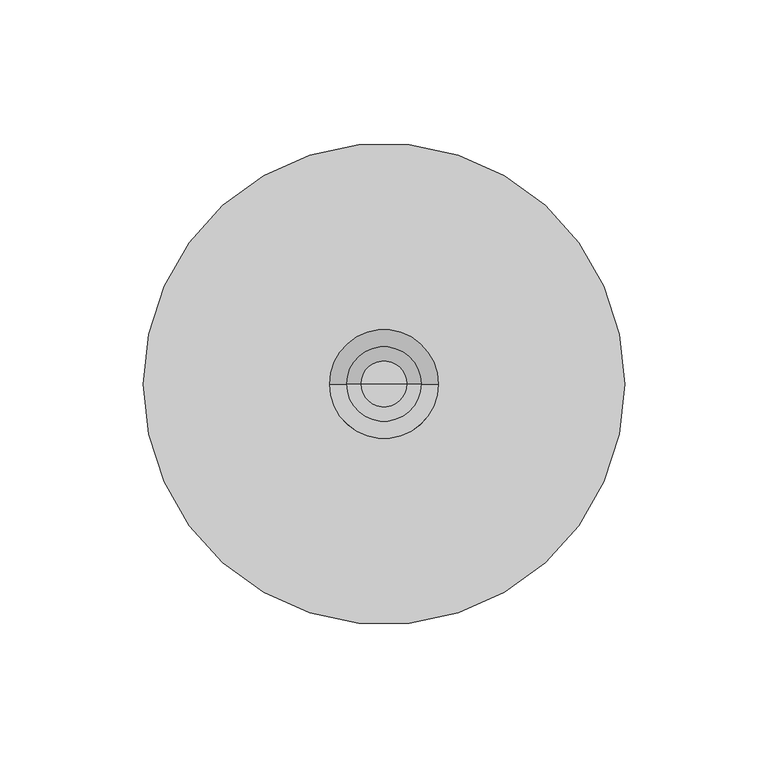
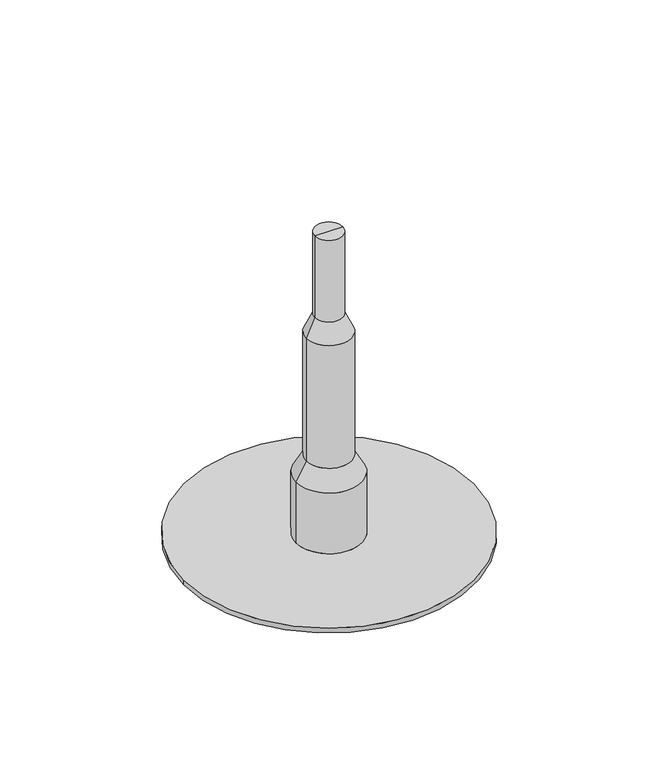
"""IFC4 building model written with IfcOpenShell, lengths in millimetres: proxy geometry, TN_Штуцер инъекционный_Прямой : ПВХ Штуцер инъекционный прямой."""

from ifc_helpers import new_model, si_unit, frame, origin, origin_with_axes, place, context, project, spatial, polyline, circle_curve, source, transform, mapped, element, save
from ifc_brep_helpers import plane_surface, cylinder_surface, revolved_surface, advanced_brep


def specialty_equipment_220ff5bd(model_context):
    return source(origin(), model_context, "Body", "AdvancedBrep", [
        advanced_brep(
        [(-19.0, 0.0, 3.0), (-19.0, 0.0, 40.0), (19.0, 0.0, 40.0), (19.0, 0.0, 3.0), (8.0, 0.0, 187.0), (-8.0, 0.0, 187.0), (0.0, 0.0, 187.0), (8.0, 0.0, 137.0), (-8.0, 0.0, 137.0), (13.0, 0.0, 126.0), (-13.0, 0.0, 126.0), (13.0, 0.0, 51.0), (-13.0, 0.0, 51.0), (-84.0, 0.0, 3.0), (84.0, 0.0, 3.0), (-84.0, 0.0, 0.0), (84.0, 0.0, 0.0)],
        [
            (0, 1),
            (1, 2, circle_curve(frame((0.0, 0.0, 40.0), z_axis=(0.0, 0.0, -1.0), x_axis=(-1.0, 0.0, 0.0)), 19.0)),
            (2, 3),
            (3, 0, circle_curve(frame((0.0, 0.0, 3.0), z_axis=(0.0, 0.0, 1.0), x_axis=(-1.0, 0.0, 0.0)), 19.0)),
            (0, 3, circle_curve(frame((0.0, 0.0, 3.0), z_axis=(0.0, 0.0, 1.0), x_axis=(-1.0, 0.0, 0.0)), 19.0)),
            (2, 1, circle_curve(frame((0.0, 0.0, 40.0), z_axis=(0.0, 0.0, -1.0), x_axis=(-1.0, 0.0, 0.0)), 19.0)),
            (4, 5, circle_curve(frame((0.0, 0.0, 187.0), z_axis=(0.0, 0.0, 1.0), x_axis=(-1.0, 0.0, 0.0)), 8.0)),
            (5, 6),
            (6, 4),
            (5, 4, circle_curve(frame((0.0, 0.0, 187.0), z_axis=(0.0, 0.0, 1.0), x_axis=(-1.0, 0.0, 0.0)), 8.0)),
            (4, 7),
            (7, 8, circle_curve(frame((0.0, 0.0, 137.0), z_axis=(0.0, 0.0, 1.0), x_axis=(-1.0, 0.0, 0.0)), 8.0)),
            (8, 5),
            (8, 7, circle_curve(frame((0.0, 0.0, 137.0), z_axis=(0.0, 0.0, 1.0), x_axis=(-1.0, 0.0, 0.0)), 8.0)),
            (7, 9),
            (9, 10, circle_curve(frame((0.0, 0.0, 126.0), z_axis=(0.0, 0.0, 1.0), x_axis=(-1.0, 0.0, 0.0)), 13.0)),
            (10, 8),
            (10, 9, circle_curve(frame((0.0, 0.0, 126.0), z_axis=(0.0, 0.0, 1.0), x_axis=(-1.0, 0.0, 0.0)), 13.0)),
            (9, 11),
            (11, 12, circle_curve(frame((0.0, 0.0, 51.0), z_axis=(0.0, 0.0, 1.0), x_axis=(-1.0, 0.0, 0.0)), 13.0)),
            (12, 10),
            (12, 11, circle_curve(frame((0.0, 0.0, 51.0), z_axis=(0.0, 0.0, 1.0), x_axis=(-1.0, 0.0, 0.0)), 13.0)),
            (1, 12),
            (11, 2),
            (13, 14, circle_curve(frame((0.0, 0.0, 3.0), z_axis=(0.0, 0.0, 1.0), x_axis=(1.0, 0.0, 0.0)), 84.0)),
            (14, 13, circle_curve(frame((0.0, 0.0, 3.0), z_axis=(0.0, 0.0, 1.0), x_axis=(1.0, 0.0, 0.0)), 84.0)),
            (15, 16, circle_curve(frame((0.0, 0.0, 0.0), z_axis=(0.0, 0.0, -1.0), x_axis=(1.0, 0.0, 0.0)), 84.0)),
            (16, 15, circle_curve(frame((0.0, 0.0, 0.0), z_axis=(0.0, 0.0, -1.0), x_axis=(1.0, 0.0, 0.0)), 84.0)),
            (13, 15),
            (16, 14),
        ],
        [
            cylinder_surface(frame((0.0, 0.0, 2214.3150031), z_axis=(0.0, 0.0, -1.0), x_axis=(-1.0, 0.0, 0.0)), 19.0),
            plane_surface(frame((0.0, 0.0, 187.0), z_axis=(0.0, 0.0, 1.0), x_axis=(-1.0, 0.0, 0.0))),
            cylinder_surface(frame((0.0, 0.0, 2214.3150031), z_axis=(0.0, 0.0, -1.0), x_axis=(-1.0, 0.0, 0.0)), 8.0),
            revolved_surface(polyline([(-8.0, 0.0, 137.0), (-13.0, 0.0, 126.0)]), (0.0, 0.0, 2214.3150031), (0.0, 0.0, -1.0)),
            cylinder_surface(frame((0.0, 0.0, 2214.3150031), z_axis=(0.0, 0.0, -1.0), x_axis=(-1.0, 0.0, 0.0)), 13.0),
            revolved_surface(polyline([(-13.0, 0.0, 51.0), (-19.0, 0.0, 40.0)]), (0.0, 0.0, 2214.3150031), (0.0, 0.0, -1.0)),
            plane_surface(frame((84.0, 0.0, 3.0), z_axis=(0.0, 0.0, 1.0), x_axis=(0.0, 1.0, 0.0))),
            plane_surface(frame((84.0, 0.0, 0.0), z_axis=(0.0, 0.0, -1.0), x_axis=(0.0, -1.0, 0.0))),
            cylinder_surface(origin_with_axes(), 84.0),
        ],
        [
            (0, [[1, 2, 3, 4]]),
            (0, [[-1, 5, -3, 6]]),
            (1, [[7, 8, 9]]),
            (1, [[-8, 10, -9]]),
            (2, [[-7, 11, 12, 13]]),
            (2, [[-10, -13, 14, -11]]),
            (3, [[-12, 15, 16, 17]]),
            (3, [[-14, -17, 18, -15]]),
            (4, [[-16, 19, 20, 21]]),
            (4, [[-18, -21, 22, -19]]),
            (5, [[-2, 23, -20, 24]]),
            (5, [[-6, -24, -22, -23]]),
            (6, [[25, 26], [-4, -5]]),
            (7, [[27, 28]]),
            (8, [[-25, 29, -28, 30]]),
            (8, [[-26, -30, -27, -29]]),
        ],
    ),
    ])


if __name__ == "__main__":
    model = new_model("IFC4")
    model_context = context("Model", 3, world=origin())
    ifc_project = project(units=[si_unit("LENGTHUNIT", "METRE", prefix="MILLI")], contexts=[model_context])
    site = spatial("IfcSite", under=ifc_project)
    building = spatial("IfcBuilding", under=site)
    placement = place(None, origin())
    specialty_equipment_shape = specialty_equipment_220ff5bd(model_context)
    element("IfcBuildingElementProxy", 1, Name="TN_Штуцер инъекционный_Прямой : ПВХ Штуцер инъекционный прямой", ObjectType="TN_Штуцер инъекционный_Прямой : ПВХ Штуцер инъекционный прямой", at=placement, inside=building, context=model_context, shape_type="MappedRepresentation", body=[
        mapped(specialty_equipment_shape, transform((0.0, 0.0, 0.0), x_axis=(1.0, 0.0, 0.0), y_axis=(0.0, 1.0, 0.0), z_axis=(0.0, 0.0, 1.0))),
    ])
    save(model, "model.ifc")

# Revit data of these elements
# Type "TN_Штуцер инъекционный_Прямой : ПВХ Штуцер инъекционный прямой"
#   Description = "Элемент инъекционной системы в составе ремонтопригодной гидроизоляционной системы на основе ПВХ мембран. Применяется для подачи ремонтного инъекционного состава к гидроизоляционной мембране."
#   Manufacturer = "ТехноНИКОЛЬ"
#   URL = "https://nav.tn.ru/catalog/gidroizolyatsiya/komplektatsiya-dlya-gidroizolyatsii/pvkh-kontrolno-inektsionnye-shtutsera/?sphrase_id=1315217"
#   ADSK_Обозначение = "ТехноНИКОЛЬ"
#   ADSK_Наименование = "ПВХ Штуцер инъекционный прямой"
#   ADSK_Код изделия = "368641"
#   ADSK_Завод-изготовитель = "ТехноНИКОЛЬ"
#   ADSK_Единица измерения = "шт."
#   ADSK_Группирование = "Штуцеры и аксессуары"
#   ADSK_URL страницы изделия = "https://nav.tn.ru/catalog/gidroizolyatsiya/komplektatsiya-dlya-gidroizolyatsii/pvkh-kontrolno-inektsionnye-shtutsera/?sphrase_id=1315217"
#   ADSK_URL документации изделия = "https://nav.tn.ru/upload/iblock/0f4/hv3xcwmq3sc3w0qtwpgcurch9nh0p8gf/21_-Tekhlist-7.70_PVKH_Kontrolno_inektsionnye-shtutsera_rus.pdf"
#   ADSK_Размер_Ширина = 168 mm
#   ADSK_Размер_Диаметр = 10 mm
#   ADSK_Размер_Высота = 187 mm
#   ADSK_Количество = 1
#   Зажим для трубки [instance default] = yes
#   Материал = TN_ПВХ_Серый
#   Default Elevation = 0
# Element 1 (IfcBuildingElementProxy, "TN_Штуцер инъекционный_Прямой : ПВХ Штуцер инъекционный прямой")
#   Materials on its faces: "TN_ПВХ_Серый"
# Materials
#   "TN_ПВХ_Серый": class "Типовые", colour RGB 192 192 192, transparency 0, Cost = 0
